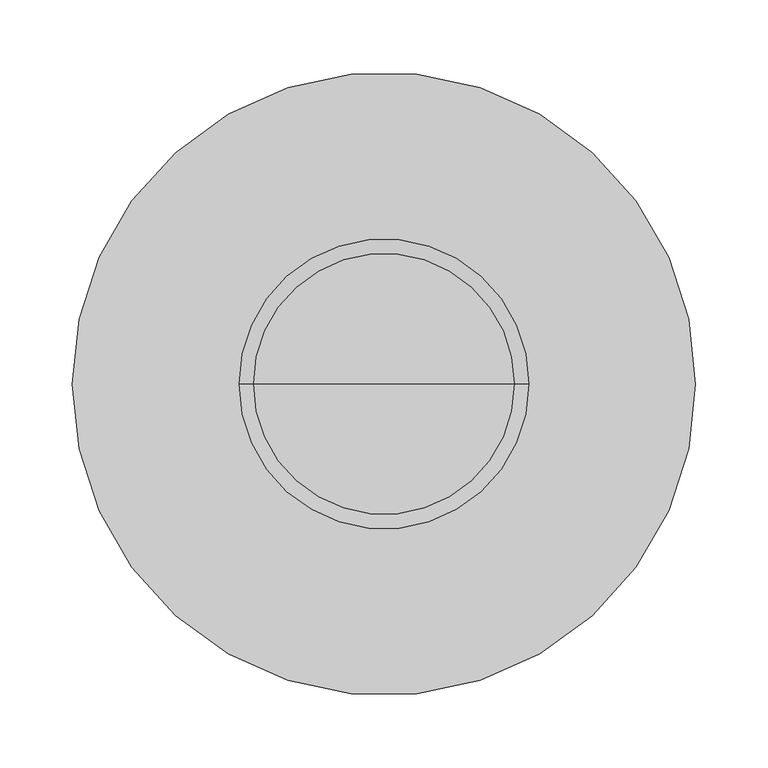
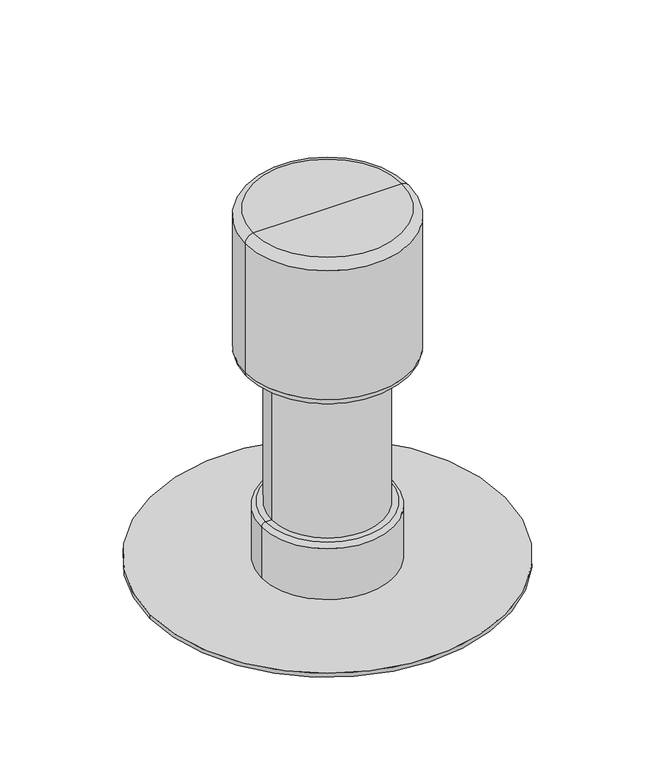
"""IFC4 building model written with IfcOpenShell, lengths in millimetres: proxy geometry, TN_Аэратор кровельный  ТехноНИКОЛЬ : Аэратор кровельный ТехноНИКОЛЬ ЭКО 160х450мм."""

from ifc_helpers import new_model, si_unit, point, frame, origin, origin_with_axes, origin_2d, place, context, project, spatial, circle_curve, ellipse_curve, trimmed, segment, composite_curve, outline, extrude, source, transform, mapped, element, save
from ifc_brep_helpers import plane_surface, cylinder_surface, revolved_surface, advanced_brep


def specialty_equipment_6541386a(model_context):
    return source(origin(), model_context, "Body", "SolidModel", [
        advanced_brep(
        [(0.0, 0.0, 5.0), (-80.0, 0.0, 5.0), (80.0, 0.0, 5.0), (67.5, 0.0, 265.0), (-67.5, 0.0, 265.0), (0.0, 0.0, 265.0), (67.5, 0.0, 75.0), (-67.5, 0.0, 75.0), (75.0, 0.0, 75.0), (-75.0, 0.0, 75.0), (80.0, 0.0, 70.0), (-80.0, 0.0, 70.0)],
        [
            (0, 1),
            (1, 2, circle_curve(frame((0.0, 0.0, 5.0), z_axis=(0.0, 0.0, -1.0), x_axis=(-1.0, 0.0, 0.0)), 80.0)),
            (2, 0),
            (2, 1, circle_curve(frame((0.0, 0.0, 5.0), z_axis=(0.0, 0.0, -1.0), x_axis=(-1.0, 0.0, 0.0)), 80.0)),
            (3, 4, circle_curve(frame((0.0, 0.0, 265.0), z_axis=(0.0, 0.0, 1.0), x_axis=(-1.0, 0.0, 0.0)), 67.5)),
            (4, 5),
            (5, 3),
            (4, 3, circle_curve(frame((0.0, 0.0, 265.0), z_axis=(0.0, 0.0, 1.0), x_axis=(-1.0, 0.0, 0.0)), 67.5)),
            (6, 7, circle_curve(frame((0.0, 0.0, 75.0), z_axis=(0.0, 0.0, 1.0), x_axis=(-1.0, 0.0, 0.0)), 67.5)),
            (7, 4),
            (3, 6),
            (7, 6, circle_curve(frame((0.0, 0.0, 75.0), z_axis=(0.0, 0.0, 1.0), x_axis=(-1.0, 0.0, 0.0)), 67.5)),
            (8, 9, circle_curve(frame((0.0, 0.0, 75.0), z_axis=(0.0, 0.0, 1.0), x_axis=(-1.0, 0.0, 0.0)), 75.0)),
            (9, 7),
            (6, 8),
            (9, 8, circle_curve(frame((0.0, 0.0, 75.0), z_axis=(0.0, 0.0, 1.0), x_axis=(-1.0, 0.0, 0.0)), 75.0)),
            (10, 11, circle_curve(frame((0.0, 0.0, 70.0), z_axis=(0.0, 0.0, 1.0), x_axis=(-1.0, 0.0, 0.0)), 80.0)),
            (11, 9, circle_curve(frame((-75.0, 0.0, 70.0), z_axis=(0.0, 1.0, 0.0), x_axis=(1.0, 0.0, 0.0)), 5.0)),
            (8, 10, circle_curve(frame((75.0, 0.0, 70.0), z_axis=(0.0, 1.0, 0.0), x_axis=(-1.0, 0.0, 0.0)), 5.0)),
            (11, 10, circle_curve(frame((0.0, 0.0, 70.0), z_axis=(0.0, 0.0, 1.0), x_axis=(-1.0, 0.0, 0.0)), 80.0)),
            (1, 11),
            (10, 2),
        ],
        [
            plane_surface(frame((0.0, 0.0, 5.0), z_axis=(0.0, 0.0, -1.0), x_axis=(-1.0, 0.0, 0.0))),
            plane_surface(frame((0.0, 0.0, 265.0), z_axis=(0.0, 0.0, 1.0), x_axis=(-1.0, 0.0, 0.0))),
            cylinder_surface(frame((0.0, 0.0, 0.0), z_axis=(0.0, 0.0, -1.0), x_axis=(-1.0, 0.0, 0.0)), 67.5),
            plane_surface(frame((0.0, 0.0, 75.0), z_axis=(0.0, 0.0, 1.0), x_axis=(-1.0, 0.0, 0.0))),
            revolved_surface(trimmed(ellipse_curve(frame((-75.0, 0.0, 70.0), z_axis=(0.0, -1.0, 0.0), x_axis=(1.0, 0.0, 0.0)), 5.0, 5.0), [point((-75.0, 0.0, 75.0))], [point((-80.0, 0.0, 70.0))], True, "CARTESIAN"), (0.0, 0.0, 0.0), (0.0, 0.0, -1.0)),
            cylinder_surface(frame((0.0, 0.0, 0.0), z_axis=(0.0, 0.0, -1.0), x_axis=(-1.0, 0.0, 0.0)), 80.0),
        ],
        [
            (0, [[1, 2, 3]]),
            (0, [[-3, 4, -1]]),
            (1, [[5, 6, 7]]),
            (1, [[8, -7, -6]]),
            (2, [[9, 10, -5, 11]]),
            (2, [[12, -11, -8, -10]]),
            (3, [[13, 14, -9, 15]]),
            (3, [[16, -15, -12, -14]]),
            (4, [[17, 18, -13, 19]]),
            (4, [[20, -19, -16, -18]]),
            (5, [[-2, 21, -17, 22]]),
            (5, [[-4, -22, -20, -21]]),
        ],
    ),
        extrude(outline(composite_curve([segment(trimmed(circle_curve(origin_2d(), 215.0), [point((-215.0, 0.0))], [point((215.0, 0.0))], False, "CARTESIAN"), True, "CONTINUOUS"), segment(trimmed(circle_curve(origin_2d(), 215.0), [point((215.0, 0.0))], [point((-215.0, 0.0))], False, "CARTESIAN"), True, "CONTINUOUS")], self_intersect=False)), origin_with_axes(), (0.0, 0.0, 1.0), 5.0),
        advanced_brep(
        [(90.0, 0.0, 450.0), (-90.0, 0.0, 450.0), (0.0, 0.0, 450.0), (100.0, 0.0, 440.0), (-100.0, 0.0, 440.0), (100.0, 0.0, 275.0), (-100.0, 0.0, 275.0), (90.0, 0.0, 265.0), (-90.0, 0.0, 265.0), (0.0, 0.0, 265.0)],
        [
            (0, 1, circle_curve(frame((0.0, 0.0, 450.0), z_axis=(0.0, 0.0, 1.0), x_axis=(-1.0, 0.0, 0.0)), 90.0)),
            (1, 2),
            (2, 0),
            (1, 0, circle_curve(frame((0.0, 0.0, 450.0), z_axis=(0.0, 0.0, 1.0), x_axis=(-1.0, 0.0, 0.0)), 90.0)),
            (3, 4, circle_curve(frame((0.0, 0.0, 440.0), z_axis=(0.0, 0.0, 1.0), x_axis=(-1.0, 0.0, 0.0)), 100.0)),
            (4, 1, circle_curve(frame((-90.0, 0.0, 440.0), z_axis=(0.0, 1.0, 0.0), x_axis=(1.0, 0.0, 0.0)), 10.0)),
            (0, 3, circle_curve(frame((90.0, 0.0, 440.0), z_axis=(0.0, 1.0, 0.0), x_axis=(-1.0, 0.0, 0.0)), 10.0)),
            (4, 3, circle_curve(frame((0.0, 0.0, 440.0), z_axis=(0.0, 0.0, 1.0), x_axis=(-1.0, 0.0, 0.0)), 100.0)),
            (5, 6, circle_curve(frame((0.0, 0.0, 275.0), z_axis=(0.0, 0.0, 1.0), x_axis=(-1.0, 0.0, 0.0)), 100.0)),
            (6, 4),
            (3, 5),
            (6, 5, circle_curve(frame((0.0, 0.0, 275.0), z_axis=(0.0, 0.0, 1.0), x_axis=(-1.0, 0.0, 0.0)), 100.0)),
            (7, 8, circle_curve(frame((0.0, 0.0, 265.0), z_axis=(0.0, 0.0, 1.0), x_axis=(-1.0, 0.0, 0.0)), 90.0)),
            (8, 6, circle_curve(frame((-90.0, 0.0, 275.0), z_axis=(0.0, 1.0, 0.0), x_axis=(1.0, 0.0, 0.0)), 10.0)),
            (5, 7, circle_curve(frame((90.0, 0.0, 275.0), z_axis=(0.0, 1.0, 0.0), x_axis=(-1.0, 0.0, 0.0)), 10.0)),
            (8, 7, circle_curve(frame((0.0, 0.0, 265.0), z_axis=(0.0, 0.0, 1.0), x_axis=(-1.0, 0.0, 0.0)), 90.0)),
            (9, 8),
            (7, 9),
        ],
        [
            plane_surface(frame((0.0, 0.0, 450.0), z_axis=(0.0, 0.0, 1.0), x_axis=(-1.0, 0.0, 0.0))),
            revolved_surface(trimmed(ellipse_curve(frame((-90.0, 0.0, 440.0), z_axis=(0.0, -1.0, 0.0), x_axis=(1.0, 0.0, 0.0)), 10.0, 10.0), [point((-90.0, 0.0, 450.0))], [point((-100.0, 0.0, 440.0))], True, "CARTESIAN"), (0.0, 0.0, 450.0), (0.0, 0.0, -1.0)),
            cylinder_surface(frame((0.0, 0.0, 450.0), z_axis=(0.0, 0.0, -1.0), x_axis=(-1.0, 0.0, 0.0)), 100.0),
            revolved_surface(trimmed(ellipse_curve(frame((-90.0, 0.0, 275.0), z_axis=(0.0, -1.0, 0.0), x_axis=(1.0, 0.0, 0.0)), 10.0, 10.0), [point((-100.0, 0.0, 275.0))], [point((-90.0, 0.0, 265.0))], True, "CARTESIAN"), (0.0, 0.0, 450.0), (0.0, 0.0, -1.0)),
            plane_surface(frame((0.0, 0.0, 265.0), z_axis=(0.0, 0.0, -1.0), x_axis=(-1.0, 0.0, 0.0))),
        ],
        [
            (0, [[1, 2, 3]]),
            (0, [[4, -3, -2]]),
            (1, [[5, 6, -1, 7]]),
            (1, [[8, -7, -4, -6]]),
            (2, [[9, 10, -5, 11]]),
            (2, [[12, -11, -8, -10]]),
            (3, [[13, 14, -9, 15]]),
            (3, [[16, -15, -12, -14]]),
            (4, [[17, -13, 18]]),
            (4, [[-18, -16, -17]]),
        ],
    ),
    ])


if __name__ == "__main__":
    model = new_model("IFC4")
    model_context = context("Model", 3, world=origin())
    ifc_project = project(units=[si_unit("LENGTHUNIT", "METRE", prefix="MILLI")], contexts=[model_context])
    site = spatial("IfcSite", under=ifc_project)
    building = spatial("IfcBuilding", under=site)
    placement = place(None, origin())
    specialty_equipment_shape = specialty_equipment_6541386a(model_context)
    element("IfcBuildingElementProxy", 1, Name="TN_Аэратор кровельный  ТехноНИКОЛЬ : Аэратор кровельный ТехноНИКОЛЬ ЭКО 160х450мм", ObjectType="TN_Аэратор кровельный  ТехноНИКОЛЬ : Аэратор кровельный ТехноНИКОЛЬ ЭКО 160х450мм", at=placement, inside=building, context=model_context, shape_type="MappedRepresentation", body=[
        mapped(specialty_equipment_shape, transform((0.0, 0.0, 0.0), x_axis=(1.0, 0.0, 0.0), y_axis=(0.0, 1.0, 0.0), z_axis=(0.0, 0.0, 1.0))),
    ])
    save(model, "model.ifc")

# Revit data of these elements
# Type "TN_Аэратор кровельный  ТехноНИКОЛЬ : Аэратор кровельный ТехноНИКОЛЬ ЭКО 160х450мм"
#   ADSK_Группирование = "Комплектующие и воронки"
#   Description = "Аэраторы кровельные ТехноНИКОЛЬ ЭКО 160х450 мм позволяют эффективно удалять излишки влаги из кровельного пирога. В системах с механическим креплением кровельного ковра к основанию рекомендуется\r\nустанавливать один аэратор на 150 м2 кровли. В кровлях устраиваемых по цементно-песчаным стяжкам с применением материалов Унифлекс ЭПВ Вент и Техноэласт ЭКВ Вент устанавливается не менее 1 аэратора на\r\n100м2. Аэраторы устанавливают равномерно по поверхности кровли. Оптимальной считается расстановка, когда большинство аэраторов установлены в местах водораздела и расстояние между аэраторами не превышает 12 м, а расстояние до паропреграждающей конструкции (парапета, деформационного шва, стены) не превышает 6м."
#   Manufacturer = "ТехноНИКОЛЬ"
#   URL = "https://shop.tn.ru/ajerator-krovel-nyj-tehnonikol-jeko-160h450-mm"
#   ADSK_Примечание = ""
#   ADSK_Обозначение = "ТехноНИКОЛЬ"
#   ADSK_Наименование = "Аэратор кровельный ТехноНИКОЛЬ ЭКО 160х450мм"
#   ADSK_Марка = ""
#   ADSK_Код изделия = "39091"
#   ADSK_Завод-изготовитель = "ТехноНИКОЛЬ"
#   ADSK_Единица измерения = "шт."
#   ADSK_Группирование = "Комплектующие и воронки"
#   ADSK_URL страницы изделия = "https://shop.tn.ru/ajerator-krovel-nyj-tehnonikol-jeko-160h450-mm"
#   ADSK_URL документации изделия = "https://nav.tn.ru/upload/iblock/68a/Tekhlist-7.18_Aerator-krovelnyy-TekhnoNIKOL_rus.pdf"
#   Диаметр юбки = 430 mm
#   Высота = 450 mm
#   ADSK_Масса = 1.5
#   ADSK_Количество = 1
#   Материал = TN_ПВХ_Коричневый
#   Default Elevation = 0
# Element 1 (IfcBuildingElementProxy, "TN_Аэратор кровельный  ТехноНИКОЛЬ : Аэратор кровельный ТехноНИКОЛЬ ЭКО 160х450мм")
#   Materials on its faces: "TN_ПВХ_Коричневый"
# Materials
#   "TN_ПВХ_Коричневый": class "Типовые", colour RGB 128 64 0, transparency 0, Cost = 0
